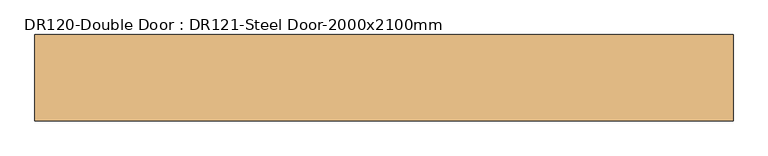
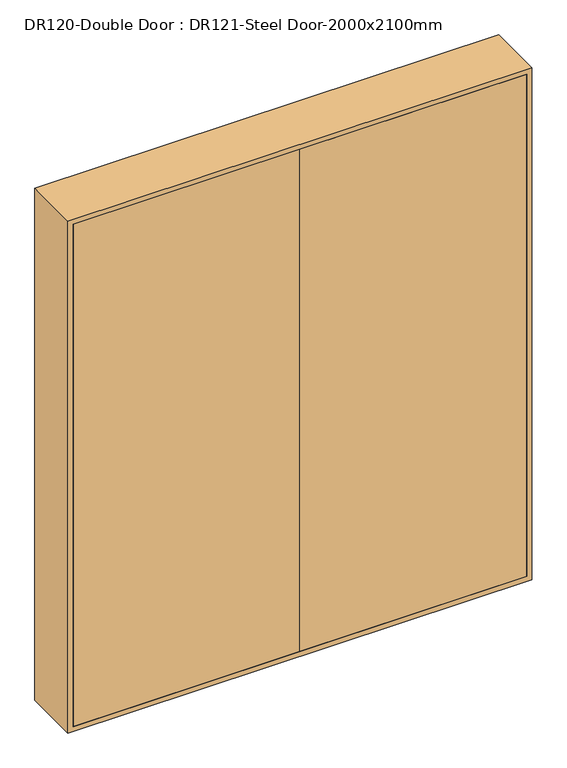
"""IFC4 building model written with IfcOpenShell, lengths in millimetres: door geometry, DR120-Double Door : DR121-Steel Door-2000x2100mm."""

from ifc_helpers import new_model, si_unit, frame, origin, place, context, project, spatial, polyline, outline, extrude, faceted_brep, source, transform, mapped, element, save


def dr120_double_door_dr121_steel_door_2000x2100mm_3724e6f2(model_context):
    return source(origin(), model_context, "Body", "SolidModel", [
        extrude(outline(polyline([(880.0, -71.0), (880.0, -111.0), (0.0, -111.0), (0.0, -71.0), (880.0, -71.0)])), frame((0.0, 0.0, 20.0), z_axis=(0.0, 0.0, 1.0), x_axis=(1.0, 0.0, 0.0)), (0.0, 0.0, 1.0), 2060.0),
        extrude(outline(polyline([(0.0, -71.0), (0.0, -111.0), (-880.0, -111.0), (-880.0, -71.0), (0.0, -71.0)])), frame((0.0, 0.0, 20.0), z_axis=(0.0, 0.0, 1.0), x_axis=(1.0, 0.0, 0.0)), (0.0, 0.0, 1.0), 2060.0),
        faceted_brep([(900.0, 111.0, 2100.0), (-900.0, 111.0, 2100.0), (-900.0, -111.0, 2100.0), (900.0, -111.0, 2100.0), (865.0, -71.0, 2065.0), (-865.0, -71.0, 2065.0), (-865.0, 111.0, 2065.0), (865.0, 111.0, 2065.0), (880.0, -111.0, 2080.0), (-880.0, -111.0, 2080.0), (-880.0, -71.0, 2080.0), (880.0, -71.0, 2080.0), (-900.0, 111.0, 0.0), (-900.0, -111.0, 0.0), (-865.0, -71.0, 35.0), (-865.0, 111.0, 35.0), (-880.0, -111.0, 20.0), (-880.0, -71.0, 20.0), (900.0, -111.0, 0.0), (880.0, -111.0, 20.0), (900.0, 111.0, 0.0), (865.0, 111.0, 35.0), (865.0, -71.0, 35.0), (880.0, -71.0, 20.0)], [[[0, 1, 2, 3]], [[4, 5, 6, 7]], [[8, 9, 10, 11]], [[1, 12, 13, 2]], [[5, 14, 15, 6]], [[9, 16, 17, 10]], [[18, 3, 2, 13], [8, 19, 16, 9]], [[12, 20, 18, 13]], [[0, 20, 12, 1], [21, 7, 6, 15]], [[14, 22, 21, 15]], [[23, 11, 10, 17], [4, 22, 14, 5]], [[16, 19, 23, 17]], [[20, 0, 3, 18]], [[22, 4, 7, 21]], [[19, 8, 11, 23]]]),
    ])


if __name__ == "__main__":
    model = new_model("IFC4")
    model_context = context("Model", 3, world=origin())
    ifc_project = project(units=[si_unit("LENGTHUNIT", "METRE", prefix="MILLI")], contexts=[model_context])
    site = spatial("IfcSite", under=ifc_project)
    building = spatial("IfcBuilding", under=site)
    placement = place(None, origin())
    dr120_double_door_dr121_steel_door_2000x2100mm_shape = dr120_double_door_dr121_steel_door_2000x2100mm_3724e6f2(model_context)
    element("IfcDoor", 1, ObjectType="DR120-Double Door : DR121-Steel Door-2000x2100mm", at=placement, inside=building, context=model_context, shape_type="MappedRepresentation", body=[
        mapped(dr120_double_door_dr121_steel_door_2000x2100mm_shape, transform((0.0, 0.0, 0.0), x_axis=(1.0, 0.0, 0.0), y_axis=(0.0, 1.0, 0.0), z_axis=(0.0, 0.0, 1.0))),
    ])
    save(model, "model.ifc")

# Revit data of these elements
# Type "DR120-Double Door : DR121-Steel Door-2000x2100mm"
#   Type Mark = "SD"
#   프레임 = ""
#   철물 = ""
#   유리/마감 = ""
#   위치/개소 = ""
#   부호 = "1/SD"
#   문번호 = ""
#   문기호 = "SD"
#   Analytic Construction = "<None>"
#   Height = 2100 mm
#   Width = 1800 mm
#   Define Thermal Properties by = 1
#   문 틀 = A04AQ098-00003_Steel Door_non FP_double
#   문 = 문
#   Function = (empty or 0)
#   Assembly Code = ""
#   Wall Closure = (empty or 0)
# Element 1 (IfcDoor, "DR120-Double Door : DR121-Steel Door-2000x2100mm")
#   Materials on its faces: "A04AQ098-00003_Steel Door_non FP_double", "문"
# Materials
#   "A04AQ098-00003_Steel Door_non FP_double": class "금속", colour RGB 247 247 247, transparency 0, Description = "Steel Door", W00) Work Master Code = "A04AQ098-00003", W01) Work Master_Lv1 = "Finishing Work", W02) Work Master_Lv2 = "Door & Window Work", W03) Work Master_Spec.1 = "Steel Door w/ Steel Frame", W04) Work Master_Spec.2 = "Fire Protective Rating: N/A, Double Door", W05) Work Master_Spec.3 = "w/ Hardware & Accessories", Cost = 0
#   "문": class "다양한", colour RGB 247 247 247, transparency 0
